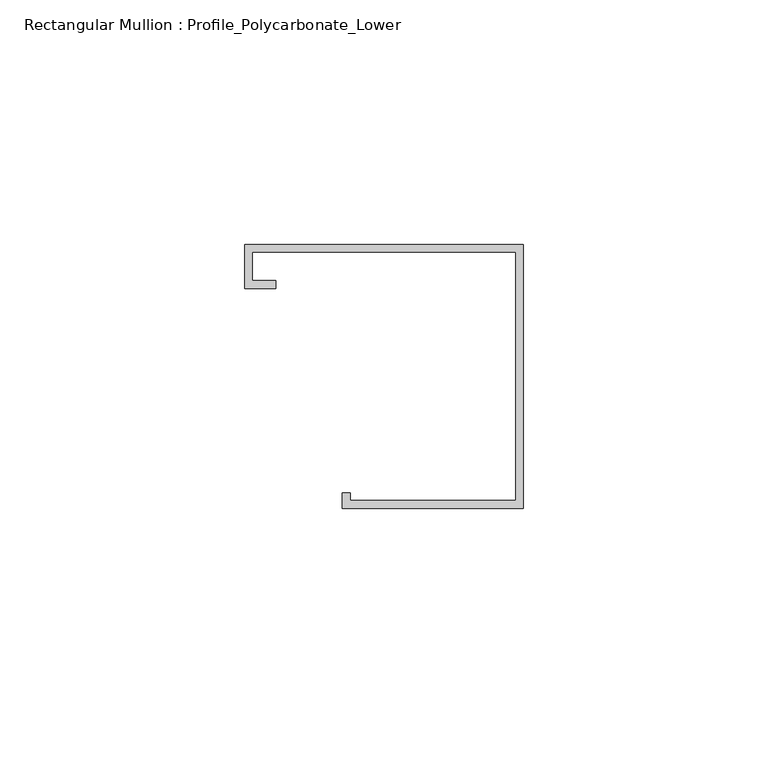
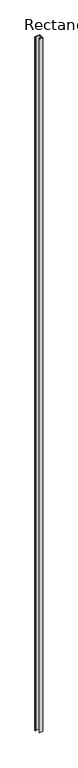
"""IFC4 building model written with IfcOpenShell, lengths in millimetres: member geometry, Rectangular Mullion : Profile_Polycarbonate_Lower."""

from ifc_helpers import new_model, si_unit, frame, origin, place, context, project, spatial, polyline, outline, extrude, source, transform, mapped, element, save


def rectangular_mullion_profile_polycarbonate_lower_33e475ce(model_context):
    return source(origin(), model_context, "Body", "SweptSolid", [
        extrude(outline(polyline([(0.0, 28.984575), (0.0, -25.015825), (-36.9824, -25.015825), (-36.9824, -21.840825), (-35.3949, -21.840825), (-35.3949, -23.428325), (-1.5875, -23.428325), (-1.5875, 27.397075), (-55.4101, 27.397075), (-55.4101, 21.580475), (-50.6476, 21.580475), (-50.6476, 19.992975), (-56.9976, 19.992975), (-56.9976, 28.984575), (0.0, 28.984575)])), frame((0.0, 0.0, -8354.1024), z_axis=(0.0, 0.0, 1.0), x_axis=(1.0, 0.0, 0.0)), (0.0, 0.0, 1.0), 8354.1024),
    ])


if __name__ == "__main__":
    model = new_model("IFC4")
    model_context = context("Model", 3, world=origin())
    ifc_project = project(units=[si_unit("LENGTHUNIT", "METRE", prefix="MILLI")], contexts=[model_context])
    site = spatial("IfcSite", under=ifc_project)
    building = spatial("IfcBuilding", under=site)
    placement = place(None, origin())
    rectangular_mullion_profile_polycarbonate_lower_shape = rectangular_mullion_profile_polycarbonate_lower_33e475ce(model_context)
    element("IfcMember", 1, ObjectType="Rectangular Mullion : Profile_Polycarbonate_Lower", at=placement, inside=building, context=model_context, shape_type="MappedRepresentation", body=[
        mapped(rectangular_mullion_profile_polycarbonate_lower_shape, transform((0.0, 0.0, 0.0), x_axis=(1.0, 0.0, 0.0), y_axis=(0.0, 1.0, 0.0), z_axis=(0.0, 0.0, 1.0))),
    ])
    save(model, "model.ifc")

# Revit data of these elements
# Type "Rectangular Mullion : Profile_Polycarbonate_Lower"
#   built-in parameter 1007322 = 0.177167 (stored number, unit not read)
#   built-in parameter 1007321 = 0 (stored number, unit not read)
#   built-in parameter 1007320 = 0.00520833 (stored number, unit not read)
